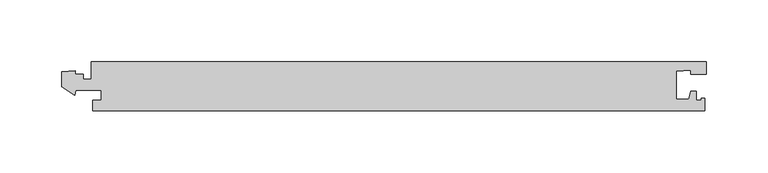
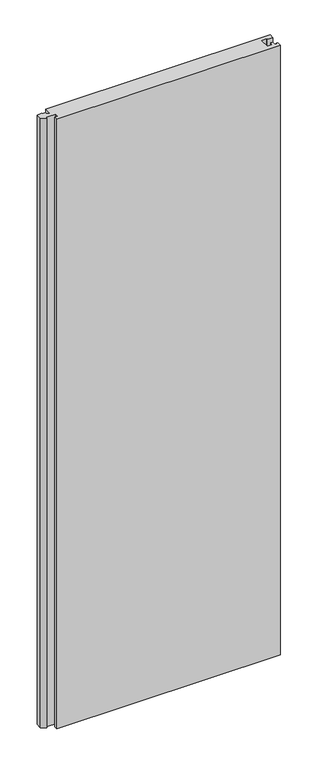
"""IFC4 building model written with IfcOpenShell, lengths in millimetres: proxy geometry, Generic Models 5:Generic Models 5:321804:Generic Models 5:321804 : Generic Models 5:Generic Models 5:321804:6 : Generic Models 5:Generic Models 5:321804:Generic Models 5:321804 : Generic Models 5:Generic Models 5:321804:300761."""

from ifc_helpers import new_model, si_unit, frame, origin, place, context, project, spatial, polyline, outline, extrude, source, transform, mapped, element, save


def generic_models_1f5e7f29(model_context):
    return source(origin(), model_context, "Body", "SweptSolid", [
        extrude(outline(polyline([(593294.8386129, -536499.5289881), (593296.5802827, -536493.0289881), (593301.0302827, -536493.0289881), (593301.0302827, -536500.5289881), (593304.9802827, -536500.5289881), (593304.9802827, -536499.0289881), (593307.9802827, -536499.0289881), (593307.9802827, -536509.0289881), (592810.4802827, -536509.0289881), (592810.4802827, -536500.5289881), (592817.4302827, -536500.5289881), (592817.4302827, -536492.5289881), (592796.7142572, -536492.5289881), (592795.6617846, -536496.4568695), (592784.9802827, -536489.3495044), (592784.9802827, -536477.4913634), (592795.9802827, -536476.5289881), (592795.9802827, -536479.2289881), (592802.6052827, -536479.2289881), (592802.6052827, -536483.5289881), (592809.2302827, -536483.5289881), (592809.2302827, -536469.0289881), (593309.2302827, -536469.0289881), (593309.2302827, -536479.2289881), (593296.4802827, -536479.2289881), (593296.4802827, -536475.9833338), (593284.4802827, -536477.0331978), (593284.4802827, -536499.5289881), (593294.8386129, -536499.5289881)])), frame((0.0, 0.0, 8611.0356611), z_axis=(0.0, 0.0, 1.0), x_axis=(1.0, 0.0, 0.0)), (0.0, 0.0, 1.0), 1435.7667058),
    ])


if __name__ == "__main__":
    model = new_model("IFC4")
    model_context = context("Model", 3, world=origin())
    ifc_project = project(units=[si_unit("LENGTHUNIT", "METRE", prefix="MILLI")], contexts=[model_context])
    site = spatial("IfcSite", under=ifc_project)
    building = spatial("IfcBuilding", under=site)
    placement = place(None, origin())
    generic_models_shape = generic_models_1f5e7f29(model_context)
    element("IfcBuildingElementProxy", 1, Name="Generic Models 5:Generic Models 5:321804:Generic Models 5:321804 : Generic Models 5:Generic Models 5:321804:6 : Generic Models 5:Generic Models 5:321804:Generic Models 5:321804 : Generic Models 5:Generic Models 5:321804:300761", ObjectType="Generic Models 5:Generic Models 5:321804:Generic Models 5:321804 : Generic Models 5:Generic Models 5:321804:6 : Generic Models 5:Generic Models 5:321804:Generic Models 5:321804 : Generic Models 5:Generic Models 5:321804:300761", at=placement, inside=building, context=model_context, shape_type="MappedRepresentation", body=[
        mapped(generic_models_shape, transform((0.0, 0.0, 0.0), x_axis=(1.0, 0.0, 0.0), y_axis=(0.0, 1.0, 0.0), z_axis=(0.0, 0.0, 1.0))),
    ])
    save(model, "model.ifc")

# Revit data of these elements
# Type "Generic Models 5:Generic Models 5:321804:Generic Models 5:321804 : Generic Models 5:Generic Models 5:321804:6 : Generic Models 5:Generic Models 5:321804:Generic Models 5:321804 : Generic Models 5:Generic Models 5:321804:300761"
#   NameOverride = "Generic Models 5:Generic Models 5:321804:Generic Models 5:321804 : Generic Models 5:Generic Models 5:321804:300761"
#   ObjectTypeOverride = "Generic Models 5:321804 : Generic Models 5:Generic Models 5:321804"
#   Reference = "Generic Models 5"
#   Tag = "300761"
# Element 1 (IfcBuildingElementProxy, "Generic Models 5:Generic Models 5:321804:Generic Models 5:321804 : Generic Models 5:Generic Models 5:321804:6 : Generic Models 5:Generic Models 5:321804:Generic Models 5:321804 : Generic Models 5:Generic Models 5:321804:300761")
#   Materials on its faces: "POLYCARBONATE PANEL - ARCOPLUS 547"
# Materials
#   "POLYCARBONATE PANEL - ARCOPLUS 547": class "Unassigned", colour RGB 202 225 249, transparency 0.45, Cost = 0
